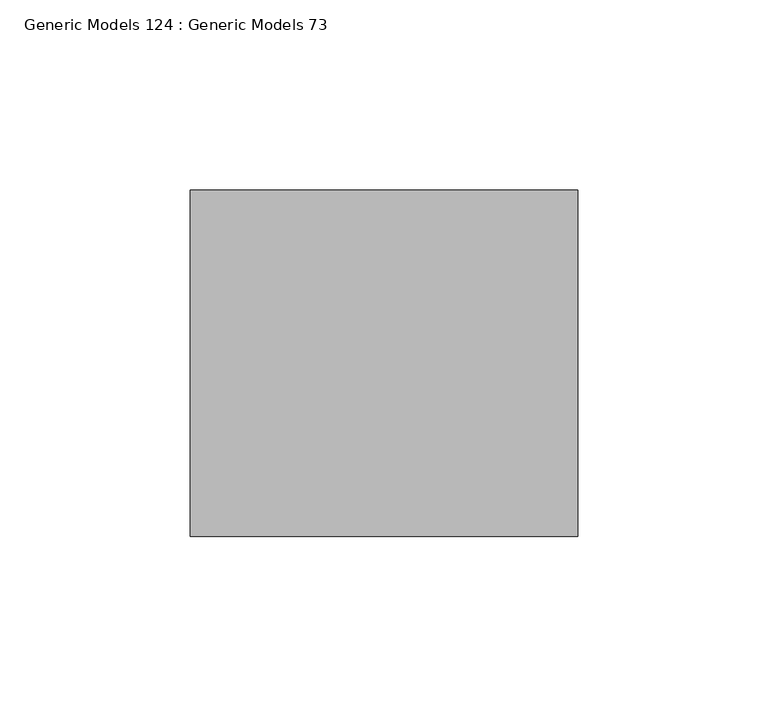
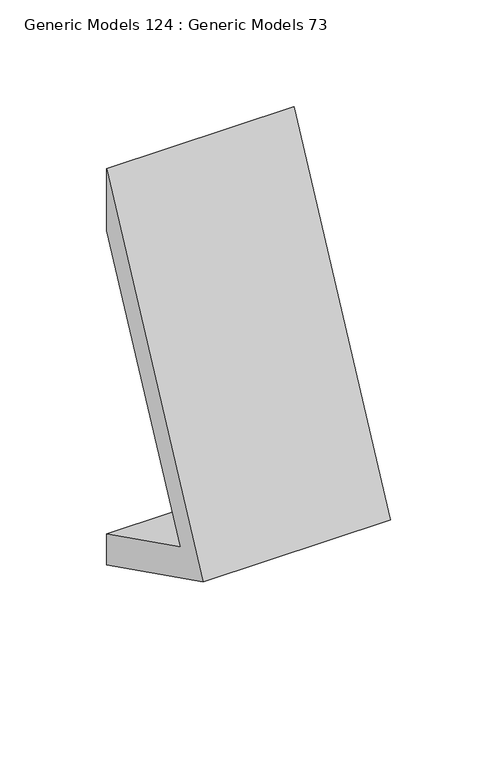
"""IFC4 building model written with IfcOpenShell, lengths in millimetres: proxy geometry, Generic Models 124 : Generic Models 73."""

from ifc_helpers import new_model, si_unit, frame, origin, place, context, project, spatial, polyline, outline, extrude, source, transform, mapped, element, save


def generic_models_124_generic_models_73_a02b07bd(model_context):
    return source(origin(), model_context, "Body", "SweptSolid", [
        extrude(outline(polyline([(35114.8094916, 269191.7744013), (35205.6832942, 269373.5220065), (35205.6832942, 269338.0244274), (35136.1080391, 269198.8739171), (35205.6832942, 269164.0862896), (35205.6832942, 269146.3375), (35114.8094916, 269191.7744013)])), frame((31924.6096032, 0.0, 0.0), z_axis=(1.0, 0.0, 0.0), x_axis=(0.0, 1.0, 0.0)), (0.0, 0.0, 1.0), 101.6),
    ])


if __name__ == "__main__":
    model = new_model("IFC4")
    model_context = context("Model", 3, world=origin())
    ifc_project = project(units=[si_unit("LENGTHUNIT", "METRE", prefix="MILLI")], contexts=[model_context])
    site = spatial("IfcSite", under=ifc_project)
    building = spatial("IfcBuilding", under=site)
    placement = place(None, origin())
    generic_models_124_generic_models_73_shape = generic_models_124_generic_models_73_a02b07bd(model_context)
    element("IfcBuildingElementProxy", 1, Name="Generic Models 124 : Generic Models 73", ObjectType="Generic Models 124 : Generic Models 73", at=placement, inside=building, context=model_context, shape_type="MappedRepresentation", body=[
        mapped(generic_models_124_generic_models_73_shape, transform((0.0, 0.0, 0.0), x_axis=(1.0, 0.0, 0.0), y_axis=(0.0, 1.0, 0.0), z_axis=(0.0, 0.0, 1.0))),
    ])
    save(model, "model.ifc")

# Revit data of these elements
# Element 1 (IfcBuildingElementProxy, "Generic Models 124 : Generic Models 73")
#   Materials on its faces: "L8 x 4 x 5/8 x 0'-4\" METAL ANGLE"
# Materials
#   "L8 x 4 x 5/8 x 0'-4\" METAL ANGLE": class "Metal", colour RGB 199 199 199, transparency 0, Description = "Carbon steel", Cost = 0
